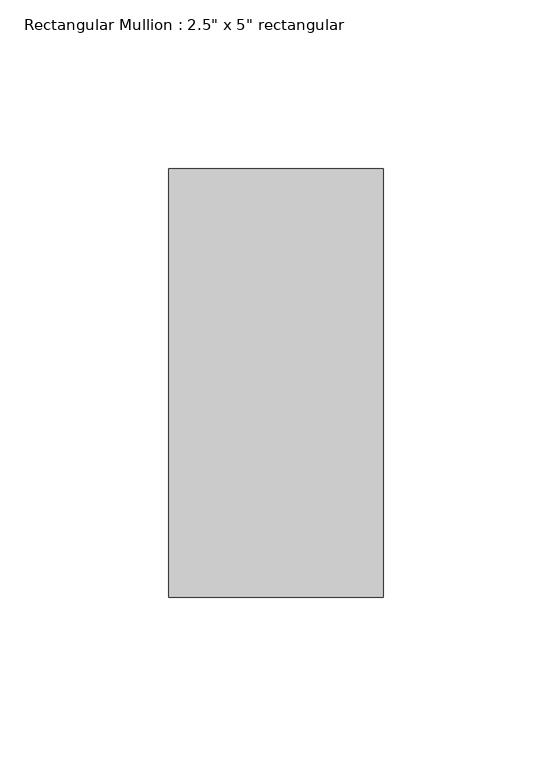
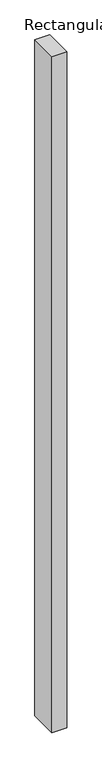
"""IFC4 building model written with IfcOpenShell, lengths in millimetres: member geometry."""

import ifcopenshell
import ifcopenshell.guid

model = None  # the IFC model being written
_history = None  # IfcOwnerHistory: only IFC2X3 demands one
_inside = {}  # id of a spatial element -> (the spatial element, [elements in it])
_under = {}  # id of a project, library or spatial element -> (it, [spatial elements below it])
_declared = {}  # id of a project -> (the project, [libraries it declares])
_typed = {}  # id of a type object -> (the type object, [elements of that type])
_made_of = {}  # id of a material, layer set ... -> (it, [elements and type objects made of it])


def new_model(schema):
    """Start an empty IFC model of exactly this schema.

    Asked for "IFC4X3", IfcOpenShell would pick the latest addendum, in which some entities
    have other attributes; the version numbers below select the first issue.
    IFC2X3 requires an IfcOwnerHistory on every rooted entity: one is made here for all.
    """
    global model, _history
    if schema == "IFC4X3":
        model = ifcopenshell.file(schema_version=(4, 3, 0, 0))
    else:
        model = ifcopenshell.file(schema=schema)
    _inside.clear()
    _under.clear()
    _declared.clear()
    _typed.clear()
    _made_of.clear()
    _history = None
    if model.schema == "IFC2X3":
        org = make("IfcOrganization", Name="unknown")
        user = make(
            "IfcPersonAndOrganization",
            ThePerson=make("IfcPerson", FamilyName="unknown"),
            TheOrganization=org,
        )
        app = make(
            "IfcApplication",
            ApplicationDeveloper=org,
            Version="unknown",
            ApplicationFullName="unknown",
            ApplicationIdentifier="unknown",
        )
        _history = make(
            "IfcOwnerHistory",
            OwningUser=user,
            OwningApplication=app,
            ChangeAction="ADDED",
            CreationDate=0,
        )
    return model


def make(cls, **values):
    """One entity of the class cls with the attributes given. An attribute that is None is left unset."""
    return model.create_entity(
        cls, **{name: value for name, value in values.items() if value is not None}
    )


def rooted(cls, **values):
    """An entity with a GlobalId (a new one), such as an element, a storey or a relation."""
    return make(cls, GlobalId=ifcopenshell.guid.new(), OwnerHistory=_history, **values)


def si_unit(unit_type, name, prefix=None):
    """IfcSIUnit, for example si_unit("LENGTHUNIT", "METRE", prefix="MILLI")."""
    return make("IfcSIUnit", UnitType=unit_type, Prefix=prefix, Name=name)


def assignment(units):
    """IfcUnitAssignment: the units of a project."""
    return None if units is None else make("IfcUnitAssignment", Units=units)


def point(xyz):
    """IfcCartesianPoint."""
    return None if xyz is None else make("IfcCartesianPoint", Coordinates=xyz)


def direction(xyz):
    """IfcDirection."""
    return None if xyz is None else make("IfcDirection", DirectionRatios=xyz)


def frame(location, z_axis=None, x_axis=None):
    """IfcAxis2Placement3D, a coordinate frame: its origin and axes. An axis left out is left unset."""
    return make(
        "IfcAxis2Placement3D",
        Location=point(location),
        Axis=direction(z_axis),
        RefDirection=direction(x_axis),
    )


def origin():
    """The frame at (0, 0, 0) with its axes left unset."""
    return frame((0.0, 0.0, 0.0))


def place(relative_to, where):
    """IfcLocalPlacement: puts the frame where relative to a parent placement (None: the world)."""
    return make(
        "IfcLocalPlacement", PlacementRelTo=relative_to, RelativePlacement=where
    )


def context(
    kind, dimensions, precision=None, world=None, true_north=None, identifier=None
):
    """IfcGeometricRepresentationContext, for example the 3D "Model" context."""
    return make(
        "IfcGeometricRepresentationContext",
        ContextIdentifier=identifier,
        ContextType=kind,
        CoordinateSpaceDimension=dimensions,
        Precision=precision,
        WorldCoordinateSystem=world,
        TrueNorth=true_north,
    )


def project(units=None, contexts=None):
    """IfcProject with its units and contexts."""
    return rooted(
        "IfcProject",
        Name="project",
        RepresentationContexts=contexts,
        UnitsInContext=assignment(units),
    )


def spatial(cls, under=None, at=None, **own):
    """A site, building, storey or space (cls), placed at a placement, below another one or the project."""
    s = rooted(cls, ObjectPlacement=at, **own)
    if under is not None:
        _under.setdefault(under.id(), (under, []))[1].append(s)
    return s


def polyline(points):
    """IfcPolyline through the points."""
    return make("IfcPolyline", Points=[point(p) for p in points])


def outline(outer, holes=None, kind="AREA"):
    """IfcArbitraryClosedProfileDef: a profile drawn as a closed curve; with holes, ...WithVoids."""
    if holes is None:
        return make("IfcArbitraryClosedProfileDef", ProfileType=kind, OuterCurve=outer)
    return make(
        "IfcArbitraryProfileDefWithVoids",
        ProfileType=kind,
        OuterCurve=outer,
        InnerCurves=holes,
    )


def extrude(swept, where, along, depth):
    """IfcExtrudedAreaSolid: the profile swept, set in the frame where, extruded along a direction by depth."""
    return make(
        "IfcExtrudedAreaSolid",
        SweptArea=swept,
        Position=where,
        ExtrudedDirection=direction(along),
        Depth=depth,
    )


def shape(context_of_items, identifier, shape_type, items):
    """IfcShapeRepresentation: the items that make up one representation, for example the "Body"."""
    return make(
        "IfcShapeRepresentation",
        ContextOfItems=context_of_items,
        RepresentationIdentifier=identifier,
        RepresentationType=shape_type,
        Items=items,
    )


def source(mapping_origin, context_of_items, identifier, shape_type, items):
    """IfcRepresentationMap: a shape defined once, which mapped items show again and again."""
    return make(
        "IfcRepresentationMap",
        MappingOrigin=mapping_origin,
        MappedRepresentation=shape(context_of_items, identifier, shape_type, items),
    )


def transform(
    local_origin,
    x_axis=None,
    y_axis=None,
    z_axis=None,
    scale=None,
    scale2=None,
    scale3=None,
    uniform=True,
):
    """IfcCartesianTransformationOperator3D, or its non-uniform kind. x_axis, y_axis, z_axis: its Axis1, 2, 3."""
    if uniform:
        return make(
            "IfcCartesianTransformationOperator3D",
            Axis1=direction(x_axis),
            Axis2=direction(y_axis),
            LocalOrigin=point(local_origin),
            Scale=scale,
            Axis3=direction(z_axis),
        )
    return make(
        "IfcCartesianTransformationOperator3DnonUniform",
        Axis1=direction(x_axis),
        Axis2=direction(y_axis),
        LocalOrigin=point(local_origin),
        Scale=scale,
        Axis3=direction(z_axis),
        Scale2=scale2,
        Scale3=scale3,
    )


def mapped(mapping_source, mapping_target):
    """IfcMappedItem: shows the shape of a source again, moved by a transform."""
    return make(
        "IfcMappedItem", MappingSource=mapping_source, MappingTarget=mapping_target
    )


def made_of(thing, what):
    """Note that an element or type object is made of a material, layer set ...; save() writes the relation."""
    if what is not None:
        _made_of.setdefault(what.id(), (what, []))[1].append(thing)
    return thing


def element(
    cls,
    number,
    at=None,
    inside=None,
    cuts=None,
    type_object=None,
    material=None,
    context=None,
    identifier="Body",
    shape_type=None,
    held_by="IfcProductDefinitionShape",
    body=None,
    shapes=None,
    **own,
):
    """One element of the class cls, such as IfcWall. Its Tag is "e" and its number.

    at: its placement. inside: the storey or other place that contains it. cuts: it is an
    opening in that element (IfcRelVoidsElement). A single representation is given by context,
    identifier, shape_type and body (its items); several are given by shapes. held_by: the class
    of the entity that holds the representations. save() writes the other relations.
    """
    e = rooted(cls, Tag="e%d" % number, ObjectPlacement=at, **own)
    if body is not None:
        shapes = [shape(context, identifier, shape_type, body)]
    if shapes is not None:
        e.Representation = make(held_by, Representations=shapes)
    if inside is not None:
        _inside.setdefault(inside.id(), (inside, []))[1].append(e)
    if cuts is not None:
        rooted(
            "IfcRelVoidsElement", RelatingBuildingElement=cuts, RelatedOpeningElement=e
        )
    if type_object is not None:
        _typed.setdefault(type_object.id(), (type_object, []))[1].append(e)
    return made_of(e, material)


def aggregate(whole, parts):
    """IfcRelAggregates: a whole, such as a stair, and the parts it consists of."""
    return rooted("IfcRelAggregates", RelatingObject=whole, RelatedObjects=parts)


def save(model, path):
    """Write the relations noted so far, then the file.

    IfcRelAggregates (storeys below a building ...), IfcRelContainedInSpatialStructure (elements
    in a storey), IfcRelDefinesByType, IfcRelAssociatesMaterial and IfcRelDeclares: one each for
    every whole, place, type object, material and project.
    """
    for whole, parts in _under.values():
        aggregate(whole, parts)
    for where, things in _inside.values():
        rooted(
            "IfcRelContainedInSpatialStructure",
            RelatedElements=things,
            RelatingStructure=where,
        )
    for kind, things in _typed.values():
        rooted("IfcRelDefinesByType", RelatedObjects=things, RelatingType=kind)
    for what, things in _made_of.values():
        rooted("IfcRelAssociatesMaterial", RelatedObjects=things, RelatingMaterial=what)
    for by, libraries in _declared.values():
        rooted("IfcRelDeclares", RelatingContext=by, RelatedDefinitions=libraries)
    model.write(path)


def member_6fa634db(model_context):
    return source(origin(), model_context, "Body", "SweptSolid", [
        extrude(outline(polyline([(31.75, 63.5), (31.75, -63.5), (-31.75, -63.5), (-31.75, 63.5), (31.75, 63.5)])), frame((0.0, 0.0, -3086.1), z_axis=(0.0, 0.0, 1.0), x_axis=(1.0, 0.0, 0.0)), (0.0, 0.0, 1.0), 3086.1),
    ])


if __name__ == "__main__":
    model = new_model("IFC4")
    model_context = context("Model", 3, world=origin())
    ifc_project = project(units=[si_unit("LENGTHUNIT", "METRE", prefix="MILLI")], contexts=[model_context])
    site = spatial("IfcSite", under=ifc_project)
    building = spatial("IfcBuilding", under=site)
    placement = place(None, origin())
    member_shape = member_6fa634db(model_context)
    element("IfcMember", 1, ObjectType="Rectangular Mullion : 2.5\" x 5\" rectangular", at=placement, inside=building, context=model_context, shape_type="MappedRepresentation", body=[
        mapped(member_shape, transform((0.0, 0.0, 0.0), x_axis=(1.0, 0.0, 0.0), y_axis=(0.0, 1.0, 0.0), z_axis=(0.0, 0.0, 1.0))),
    ])
    save(model, "model.ifc")

# Revit data of these elements
# Type "Rectangular Mullion : 2.5\" x 5\" rectangular"
#   built-in parameter 1007304 = 0.416667 (stored number, unit not read)
#   built-in parameter 1007301 = 0.104167 (stored number, unit not read)
#   built-in parameter 1007300 = 0.104167 (stored number, unit not read)
# Element 1 (IfcMember, "Rectangular Mullion : 2.5\" x 5\" rectangular")
#   Materials on its faces: "Aluminum"
# Materials
#   "Aluminum": class "Metal", colour RGB 247 247 247, transparency 0, Description = "Aluminum 6061", Cost = 0
